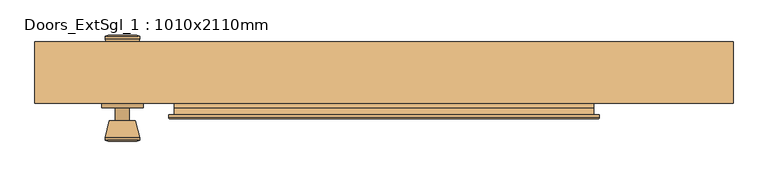
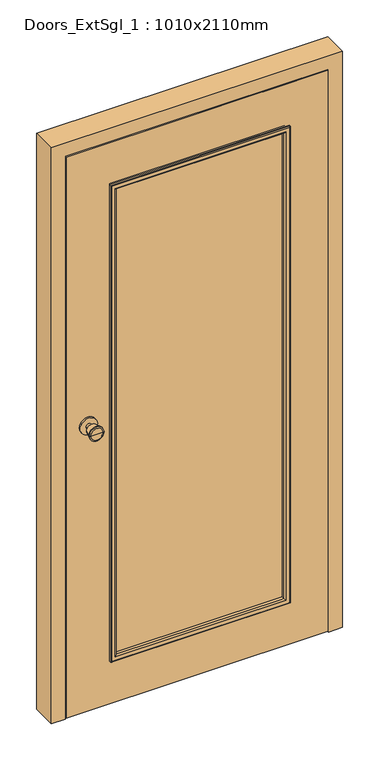
"""IFC4 building model written with IfcOpenShell, lengths in millimetres: door geometry, Doors_ExtSgl_1 : 1010x2110mm."""

from ifc_helpers import new_model, si_unit, point, frame, frame_2d, origin, place, context, project, spatial, polyline, circle_curve, ellipse_curve, trimmed, segment, composite_curve, outline, extrude, faceted_brep, source, transform, mapped, element, save
from ifc_brep_helpers import plane_surface, cylinder_surface, revolved_surface, advanced_brep


def doors_extsgl_1_1010x2110mm_099c12f8(model_context):
    return source(origin(), model_context, "Body", "SolidModel", [
        advanced_brep(
        [(-378.5, 46.25, 1050.0), (-368.5, 46.25, 1050.0), (-388.5, 46.25, 1050.0), (-358.0241324, -2.75, 1050.0), (-378.5, -2.75, 1050.0), (-398.9758676, -2.75, 1050.0), (-353.5, -0.9221319, 1050.0), (-403.5, -0.9221319, 1050.0), (-353.5, 2.5415463, 1050.0), (-403.5, 2.5415463, 1050.0), (-359.863764, 27.25, 1050.0), (-397.136236, 27.25, 1050.0), (-368.5, 27.25, 1050.0), (-388.5, 27.25, 1050.0)],
        [
            (0, 1),
            (1, 2, circle_curve(frame((-378.5, 46.25, 1050.0), z_axis=(0.0, 1.0, 0.0), x_axis=(-1.0, 0.0, 0.0)), 10.0)),
            (2, 0),
            (2, 1, circle_curve(frame((-378.5, 46.25, 1050.0), z_axis=(0.0, 1.0, 0.0), x_axis=(-1.0, 0.0, 0.0)), 10.0)),
            (3, 4),
            (4, 5),
            (5, 3, circle_curve(frame((-378.5, -2.75, 1050.0), z_axis=(0.0, -1.0, 0.0), x_axis=(-1.0, 0.0, 0.0)), 20.4758676)),
            (3, 5, circle_curve(frame((-378.5, -2.75, 1050.0), z_axis=(0.0, -1.0, 0.0), x_axis=(-1.0, 0.0, 0.0)), 20.4758676)),
            (6, 3),
            (5, 7),
            (7, 6, circle_curve(frame((-378.5, -0.9221319, 1050.0), z_axis=(0.0, -1.0, 0.0), x_axis=(-1.0, 0.0, 0.0)), 25.0)),
            (6, 7, circle_curve(frame((-378.5, -0.9221319, 1050.0), z_axis=(0.0, -1.0, 0.0), x_axis=(-1.0, 0.0, 0.0)), 25.0)),
            (8, 6),
            (7, 9),
            (9, 8, circle_curve(frame((-378.5, 2.5415463, 1050.0), z_axis=(0.0, -1.0, 0.0), x_axis=(-1.0, 0.0, 0.0)), 25.0)),
            (8, 9, circle_curve(frame((-378.5, 2.5415463, 1050.0), z_axis=(0.0, -1.0, 0.0), x_axis=(-1.0, 0.0, 0.0)), 25.0)),
            (10, 8),
            (9, 11),
            (11, 10, circle_curve(frame((-378.5, 27.25, 1050.0), z_axis=(0.0, -1.0, 0.0), x_axis=(-1.0, 0.0, 0.0)), 18.636236)),
            (10, 11, circle_curve(frame((-378.5, 27.25, 1050.0), z_axis=(0.0, -1.0, 0.0), x_axis=(-1.0, 0.0, 0.0)), 18.636236)),
            (12, 10),
            (11, 13),
            (13, 12, circle_curve(frame((-378.5, 27.25, 1050.0), z_axis=(0.0, -1.0, 0.0), x_axis=(-1.0, 0.0, 0.0)), 10.0)),
            (12, 13, circle_curve(frame((-378.5, 27.25, 1050.0), z_axis=(0.0, -1.0, 0.0), x_axis=(-1.0, 0.0, 0.0)), 10.0)),
            (1, 12),
            (13, 2),
        ],
        [
            plane_surface(frame((-378.5, 46.25, 1050.0), z_axis=(0.0, 1.0, 0.0), x_axis=(-1.0, 0.0, 0.0))),
            plane_surface(frame((-378.5, -2.75, 1050.0), z_axis=(0.0, -1.0, 0.0), x_axis=(-1.0, 0.0, 0.0))),
            revolved_surface(polyline([(-398.9758676, -2.75, 1050.0), (-403.5, -0.9221319, 1050.0)]), (-378.5, 46.25, 1050.0), (0.0, 1.0, 0.0)),
            cylinder_surface(frame((-378.5, 46.25, 1050.0), z_axis=(0.0, 1.0, 0.0), x_axis=(-1.0, 0.0, 0.0)), 25.0),
            revolved_surface(polyline([(-403.5, 2.5415463, 1050.0), (-397.136236, 27.25, 1050.0)]), (-378.5, 46.25, 1050.0), (0.0, 1.0, 0.0)),
            plane_surface(frame((-378.5, 27.25, 1050.0), z_axis=(0.0, 1.0, 0.0), x_axis=(-1.0, 0.0, 0.0))),
            cylinder_surface(frame((-378.5, 46.25, 1050.0), z_axis=(0.0, 1.0, 0.0), x_axis=(-1.0, 0.0, 0.0)), 10.0),
        ],
        [
            (0, [[1, 2, 3]]),
            (0, [[-3, 4, -1]]),
            (1, [[5, 6, 7]]),
            (1, [[-6, -5, 8]]),
            (2, [[9, -7, 10, 11]]),
            (2, [[-10, -8, -9, 12]]),
            (3, [[13, -11, 14, 15]]),
            (3, [[-14, -12, -13, 16]]),
            (4, [[17, -15, 18, 19]]),
            (4, [[-18, -16, -17, 20]]),
            (5, [[21, -19, 22, 23]]),
            (5, [[-22, -20, -21, 24]]),
            (6, [[25, -23, 26, -2]]),
            (6, [[-26, -24, -25, -4]]),
        ],
    ),
        extrude(outline(composite_curve([segment(trimmed(circle_curve(frame_2d((1050.0, -378.5)), 30.0), [point((1050.0, -408.5))], [point((1050.0, -348.5))], False, "CARTESIAN"), True, "CONTINUOUS"), segment(trimmed(circle_curve(frame_2d((1050.0, -378.5)), 30.0), [point((1050.0, -348.5))], [point((1050.0, -408.5))], False, "CARTESIAN"), True, "CONTINUOUS")], self_intersect=False)), frame((0.0, 46.25, 0.0), z_axis=(0.0, 1.0, 0.0), x_axis=(0.0, 0.0, 1.0)), (0.0, 0.0, 1.0), 6.0),
        advanced_brep(
        [(-378.5, 102.25, 1050.0), (-388.5, 102.25, 1050.0), (-368.5, 102.25, 1050.0), (-358.0241324, 151.25, 1050.0), (-398.9758676, 151.25, 1050.0), (-378.5, 151.25, 1050.0), (-353.5, 149.4221319, 1050.0), (-403.5, 149.4221319, 1050.0), (-353.5, 145.9584537, 1050.0), (-403.5, 145.9584537, 1050.0), (-359.863764, 121.25, 1050.0), (-397.136236, 121.25, 1050.0), (-368.5, 121.25, 1050.0), (-388.5, 121.25, 1050.0)],
        [
            (0, 1),
            (1, 2, circle_curve(frame((-378.5, 102.25, 1050.0), z_axis=(0.0, -1.0, 0.0), x_axis=(-1.0, 0.0, 0.0)), 10.0)),
            (2, 0),
            (2, 1, circle_curve(frame((-378.5, 102.25, 1050.0), z_axis=(0.0, -1.0, 0.0), x_axis=(-1.0, 0.0, 0.0)), 10.0)),
            (3, 4, circle_curve(frame((-378.5, 151.25, 1050.0), z_axis=(0.0, 1.0, 0.0), x_axis=(-1.0, 0.0, 0.0)), 20.4758676)),
            (4, 5),
            (5, 3),
            (4, 3, circle_curve(frame((-378.5, 151.25, 1050.0), z_axis=(0.0, 1.0, 0.0), x_axis=(-1.0, 0.0, 0.0)), 20.4758676)),
            (6, 7, circle_curve(frame((-378.5, 149.4221319, 1050.0), z_axis=(0.0, 1.0, 0.0), x_axis=(-1.0, 0.0, 0.0)), 25.0)),
            (7, 4),
            (3, 6),
            (7, 6, circle_curve(frame((-378.5, 149.4221319, 1050.0), z_axis=(0.0, 1.0, 0.0), x_axis=(-1.0, 0.0, 0.0)), 25.0)),
            (8, 9, circle_curve(frame((-378.5, 145.9584537, 1050.0), z_axis=(0.0, 1.0, 0.0), x_axis=(-1.0, 0.0, 0.0)), 25.0)),
            (9, 7),
            (6, 8),
            (9, 8, circle_curve(frame((-378.5, 145.9584537, 1050.0), z_axis=(0.0, 1.0, 0.0), x_axis=(-1.0, 0.0, 0.0)), 25.0)),
            (10, 11, circle_curve(frame((-378.5, 121.25, 1050.0), z_axis=(0.0, 1.0, 0.0), x_axis=(-1.0, 0.0, 0.0)), 18.636236)),
            (11, 9),
            (8, 10),
            (11, 10, circle_curve(frame((-378.5, 121.25, 1050.0), z_axis=(0.0, 1.0, 0.0), x_axis=(-1.0, 0.0, 0.0)), 18.636236)),
            (12, 13, circle_curve(frame((-378.5, 121.25, 1050.0), z_axis=(0.0, 1.0, 0.0), x_axis=(-1.0, 0.0, 0.0)), 10.0)),
            (13, 11),
            (10, 12),
            (13, 12, circle_curve(frame((-378.5, 121.25, 1050.0), z_axis=(0.0, 1.0, 0.0), x_axis=(-1.0, 0.0, 0.0)), 10.0)),
            (1, 13),
            (12, 2),
        ],
        [
            plane_surface(frame((-378.5, 102.25, 1050.0), z_axis=(0.0, -1.0, 0.0), x_axis=(-1.0, 0.0, 0.0))),
            plane_surface(frame((-378.5, 151.25, 1050.0), z_axis=(0.0, 1.0, 0.0), x_axis=(-1.0, 0.0, 0.0))),
            revolved_surface(polyline([(-398.9758676, 151.25, 1050.0), (-403.5, 149.4221319, 1050.0)]), (-378.5, 102.25, 1050.0), (0.0, -1.0, 0.0)),
            cylinder_surface(frame((-378.5, 102.25, 1050.0), z_axis=(0.0, -1.0, 0.0), x_axis=(-1.0, 0.0, 0.0)), 25.0),
            revolved_surface(polyline([(-403.5, 145.9584537, 1050.0), (-397.136236, 121.25, 1050.0)]), (-378.5, 102.25, 1050.0), (0.0, -1.0, 0.0)),
            plane_surface(frame((-378.5, 121.25, 1050.0), z_axis=(0.0, -1.0, 0.0), x_axis=(-1.0, 0.0, 0.0))),
            cylinder_surface(frame((-378.5, 102.25, 1050.0), z_axis=(0.0, -1.0, 0.0), x_axis=(-1.0, 0.0, 0.0)), 10.0),
        ],
        [
            (0, [[1, 2, 3]]),
            (0, [[-3, 4, -1]]),
            (1, [[5, 6, 7]]),
            (1, [[8, -7, -6]]),
            (2, [[9, 10, -5, 11]]),
            (2, [[12, -11, -8, -10]]),
            (3, [[13, 14, -9, 15]]),
            (3, [[16, -15, -12, -14]]),
            (4, [[17, 18, -13, 19]]),
            (4, [[20, -19, -16, -18]]),
            (5, [[21, 22, -17, 23]]),
            (5, [[24, -23, -20, -22]]),
            (6, [[-2, 25, -21, 26]]),
            (6, [[-4, -26, -24, -25]]),
        ],
    ),
        extrude(outline(composite_curve([segment(trimmed(circle_curve(frame_2d((1050.0, -378.5)), 30.0), [point((1050.0, -408.5))], [point((1050.0, -348.5))], False, "CARTESIAN"), True, "CONTINUOUS"), segment(trimmed(circle_curve(frame_2d((1050.0, -378.5)), 30.0), [point((1050.0, -348.5))], [point((1050.0, -408.5))], False, "CARTESIAN"), True, "CONTINUOUS")], self_intersect=False)), frame((0.0, 96.25, 0.0), z_axis=(0.0, 1.0, 0.0), x_axis=(0.0, 0.0, 1.0)), (0.0, 0.0, 1.0), 6.0),
        faceted_brep([(434.5, 141.25, 0.0), (505.0, 141.25, 0.0), (505.0, 52.25, 0.0), (456.5, 52.25, 0.0), (456.5, 99.25, 0.0), (434.5, 99.25, 0.0), (434.5, 141.25, 2039.5), (-434.5, 141.25, 2039.5), (-434.5, 141.25, 0.0), (-505.0, 141.25, 0.0), (-505.0, 141.25, 2110.0), (505.0, 141.25, 2110.0), (505.0, 52.25, 2110.0), (-505.0, 52.25, 2110.0), (-505.0, 52.25, 0.0), (-456.5, 52.25, 0.0), (-456.5, 52.25, 2061.5), (456.5, 52.25, 2061.5), (456.5, 99.25, 2061.5), (-456.5, 99.25, 2061.5), (-456.5, 99.25, 0.0), (-434.5, 99.25, 0.0), (-434.5, 99.25, 2039.5), (434.5, 99.25, 2039.5)], [[[0, 1, 2, 3, 4, 5]], [[1, 0, 6, 7, 8, 9, 10, 11]], [[2, 1, 11, 12]], [[3, 2, 12, 13, 14, 15, 16, 17]], [[4, 3, 17, 18]], [[5, 4, 18, 19, 20, 21, 22, 23]], [[0, 5, 23, 6]], [[7, 22, 21, 8]], [[8, 21, 20, 15, 14, 9]], [[13, 10, 9, 14]], [[19, 16, 15, 20]], [[12, 11, 10, 13]], [[18, 17, 16, 19]], [[6, 23, 22, 7]]]),
        extrude(outline(polyline([(-303.5, 70.0), (303.5, 70.0), (303.5, 46.0), (-303.5, 46.0), (-303.5, 70.0)])), frame((0.0, 0.0, 179.0), z_axis=(0.0, 0.0, 1.0), x_axis=(1.0, 0.0, 0.0)), (0.0, 0.0, 1.0), 1729.5),
        extrude(outline(polyline([(4.0, 453.5), (2058.5, 453.5), (2058.5, -454.4250294), (4.0, -454.4250294), (4.0, 453.5)]), holes=[polyline([(179.0, -303.5), (1908.5, -303.5), (1908.5, 303.5), (179.0, 303.5), (179.0, -303.5)])]), frame((0.0, 52.25, 0.0), z_axis=(0.0, 1.0, 0.0), x_axis=(0.0, 0.0, 1.0)), (0.0, 0.0, 1.0), 44.0),
        advanced_brep(
        [(311.5, 32.0, 171.0), (311.5, 36.0, 171.0), (311.5, 36.0, 1916.5), (311.5, 32.0, 1916.5), (309.5, 30.0, 173.0), (309.5, 30.0, 1914.5), (291.5, 35.0, 191.0), (296.5, 30.0, 186.0), (296.5, 30.0, 1901.5), (291.5, 35.0, 1896.5), (291.5, 46.0, 191.0), (291.5, 46.0, 1896.5), (303.5, 36.0, 179.0), (303.5, 46.0, 179.0), (303.5, 46.0, 1908.5), (303.5, 36.0, 1908.5), (-311.5, 36.0, 1916.5), (-311.5, 32.0, 1916.5), (-309.5, 30.0, 1914.5), (-296.5, 30.0, 1901.5), (-291.5, 35.0, 1896.5), (-291.5, 46.0, 1896.5), (-303.5, 46.0, 1908.5), (-303.5, 36.0, 1908.5), (-311.5, 36.0, 171.0), (-311.5, 32.0, 171.0), (-309.5, 30.0, 173.0), (-296.5, 30.0, 186.0), (-291.5, 35.0, 191.0), (-291.5, 46.0, 191.0), (-303.5, 46.0, 179.0), (-303.5, 36.0, 179.0)],
        [
            (0, 1),
            (1, 2),
            (2, 3),
            (3, 0),
            (4, 0, ellipse_curve(frame((309.5, 32.0, 173.0), z_axis=(0.7071067811865475, 0.0, 0.7071067811865476), x_axis=(0.7071067811865476, 0.0, -0.7071067811865475)), 2.8284271, 2.0)),
            (3, 5, ellipse_curve(frame((309.5, 32.0, 1914.5), z_axis=(0.7071067811865475, 0.0, -0.7071067811865475), x_axis=(-0.7071067811865474, 0.0, -0.7071067811865476)), 2.8284271, 2.0)),
            (5, 4),
            (6, 7, ellipse_curve(frame((296.5, 35.0, 186.0), z_axis=(0.7071067811865475, 0.0, 0.7071067811865476), x_axis=(0.7071067811865476, 0.0, -0.7071067811865475)), 7.0710678, 5.0)),
            (7, 8),
            (8, 9, ellipse_curve(frame((296.5, 35.0, 1901.5), z_axis=(0.7071067811865475, 0.0, -0.7071067811865475), x_axis=(-0.7071067811865474, 0.0, -0.7071067811865476)), 7.0710678, 5.0)),
            (9, 6),
            (10, 6),
            (9, 11),
            (11, 10),
            (12, 13),
            (13, 14),
            (14, 15),
            (15, 12),
            (2, 16),
            (16, 17),
            (17, 3),
            (17, 18, ellipse_curve(frame((-309.5, 32.0, 1914.5), z_axis=(0.7071067811865476, 0.0, 0.7071067811865475), x_axis=(0.7071067811865474, 0.0, -0.7071067811865476)), 2.8284271, 2.0)),
            (18, 5),
            (8, 19),
            (19, 20, ellipse_curve(frame((-296.5, 35.0, 1901.5), z_axis=(0.7071067811865476, 0.0, 0.7071067811865475), x_axis=(0.7071067811865474, 0.0, -0.7071067811865476)), 7.0710678, 5.0)),
            (20, 9),
            (20, 21),
            (21, 11),
            (14, 22),
            (22, 23),
            (23, 15),
            (16, 24),
            (24, 25),
            (25, 17),
            (25, 26, ellipse_curve(frame((-309.5, 32.0, 173.0), z_axis=(-0.7071067811865475, 0.0, 0.7071067811865475), x_axis=(0.7071067811865474, 0.0, 0.7071067811865476)), 2.8284271, 2.0)),
            (26, 18),
            (19, 27),
            (27, 28, ellipse_curve(frame((-296.5, 35.0, 186.0), z_axis=(-0.7071067811865475, 0.0, 0.7071067811865475), x_axis=(0.7071067811865474, 0.0, 0.7071067811865476)), 7.0710678, 5.0)),
            (28, 20),
            (28, 29),
            (29, 21),
            (22, 30),
            (30, 31),
            (31, 23),
            (24, 1),
            (0, 25),
            (4, 26),
            (7, 27),
            (6, 28),
            (10, 29),
            (13, 30),
            (12, 31),
        ],
        [
            plane_surface(frame((311.5, 36.0, 171.0), z_axis=(1.0, 0.0, 0.0), x_axis=(0.0, 0.0, 1.0))),
            cylinder_surface(frame((309.5, 32.0, 179.0), z_axis=(0.0, 0.0, -1.0), x_axis=(1.0, 0.0, 0.0)), 2.0),
            cylinder_surface(frame((296.5, 35.0, 179.0), z_axis=(0.0, 0.0, -1.0), x_axis=(1.0, 0.0, 0.0)), 5.0),
            plane_surface(frame((291.5, 35.0, 191.0), z_axis=(-1.0, 0.0, 0.0), x_axis=(0.0, 0.0, 1.0))),
            plane_surface(frame((303.5, 46.0, 179.0), z_axis=(1.0, 0.0, 0.0), x_axis=(0.0, 0.0, 1.0))),
            plane_surface(frame((311.5, 36.0, 1916.5), z_axis=(0.0, 0.0, 1.0), x_axis=(-1.0, 0.0, 0.0))),
            cylinder_surface(frame((303.5, 32.0, 1914.5), z_axis=(1.0, 0.0, 0.0), x_axis=(0.0, 0.0, 1.0)), 2.0),
            cylinder_surface(frame((303.5, 35.0, 1901.5), z_axis=(1.0, 0.0, 0.0), x_axis=(0.0, 0.0, 1.0)), 5.0),
            plane_surface(frame((291.5, 35.0, 1896.5), z_axis=(0.0, 0.0, -1.0), x_axis=(-1.0, 0.0, 0.0))),
            plane_surface(frame((303.5, 46.0, 1908.5), z_axis=(0.0, 0.0, 1.0), x_axis=(-1.0, 0.0, 0.0))),
            plane_surface(frame((-311.5, 36.0, 1916.5), z_axis=(-1.0, 0.0, 0.0), x_axis=(0.0, 0.0, -1.0))),
            cylinder_surface(frame((-309.5, 32.0, 1908.5), z_axis=(0.0, 0.0, 1.0), x_axis=(-1.0, 0.0, 0.0)), 2.0),
            cylinder_surface(frame((-296.5, 35.0, 1908.5), z_axis=(0.0, 0.0, 1.0), x_axis=(-1.0, 0.0, 0.0)), 5.0),
            plane_surface(frame((-291.5, 35.0, 1896.5), z_axis=(1.0, 0.0, 0.0), x_axis=(0.0, 0.0, -1.0))),
            plane_surface(frame((-303.5, 46.0, 1908.5), z_axis=(-1.0, 0.0, 0.0), x_axis=(0.0, 0.0, -1.0))),
            plane_surface(frame((-311.5, 36.0, 171.0), z_axis=(0.0, 0.0, -1.0), x_axis=(1.0, 0.0, 0.0))),
            cylinder_surface(frame((-303.5, 32.0, 173.0), z_axis=(-1.0, 0.0, 0.0), x_axis=(0.0, 0.0, -1.0)), 2.0),
            plane_surface(frame((-309.5, 30.0, 173.0), z_axis=(0.0, -1.0, 0.0), x_axis=(1.0, 0.0, 0.0))),
            cylinder_surface(frame((-303.5, 35.0, 186.0), z_axis=(-1.0, 0.0, 0.0), x_axis=(0.0, 0.0, -1.0)), 5.0),
            plane_surface(frame((-291.5, 35.0, 191.0), z_axis=(0.0, 0.0, 1.0), x_axis=(1.0, 0.0, 0.0))),
            plane_surface(frame((-291.5, 46.0, 191.0), z_axis=(0.0, 1.0, 0.0), x_axis=(1.0, 0.0, 0.0))),
            plane_surface(frame((-303.5, 46.0, 179.0), z_axis=(0.0, 0.0, -1.0), x_axis=(1.0, 0.0, 0.0))),
            plane_surface(frame((-303.5, 36.0, 179.0), z_axis=(0.0, 1.0, 0.0), x_axis=(1.0, 0.0, 0.0))),
        ],
        [
            (0, [[1, 2, 3, 4]]),
            (1, [[5, -4, 6, 7]]),
            (2, [[8, 9, 10, 11]]),
            (3, [[12, -11, 13, 14]]),
            (4, [[15, 16, 17, 18]]),
            (5, [[-3, 19, 20, 21]]),
            (6, [[-6, -21, 22, 23]]),
            (7, [[-10, 24, 25, 26]]),
            (8, [[-13, -26, 27, 28]]),
            (9, [[-17, 29, 30, 31]]),
            (10, [[-20, 32, 33, 34]]),
            (11, [[-22, -34, 35, 36]]),
            (12, [[-25, 37, 38, 39]]),
            (13, [[-27, -39, 40, 41]]),
            (14, [[-30, 42, 43, 44]]),
            (15, [[-33, 45, -1, 46]]),
            (16, [[-35, -46, -5, 47]]),
            (17, [[-23, -36, -47, -7], [48, -37, -24, -9]]),
            (18, [[-38, -48, -8, 49]]),
            (19, [[-40, -49, -12, 50]]),
            (20, [[51, -42, -29, -16], [-28, -41, -50, -14]]),
            (21, [[-43, -51, -15, 52]]),
            (22, [[-45, -32, -19, -2], [-31, -44, -52, -18]]),
        ],
    ),
        advanced_brep(
        [(-311.5, 84.0, 171.0), (-311.5, 80.0, 171.0), (-311.5, 80.0, 1916.5), (-311.5, 84.0, 1916.5), (-309.5, 86.0, 173.0), (-309.5, 86.0, 1914.5), (-291.5, 81.0, 191.0), (-296.5, 86.0, 186.0), (-296.5, 86.0, 1901.5), (-291.5, 81.0, 1896.5), (-291.5, 70.0, 191.0), (-291.5, 70.0, 1896.5), (-303.5, 80.0, 179.0), (-303.5, 70.0, 179.0), (-303.5, 70.0, 1908.5), (-303.5, 80.0, 1908.5), (311.5, 80.0, 1916.5), (311.5, 84.0, 1916.5), (309.5, 86.0, 1914.5), (296.5, 86.0, 1901.5), (291.5, 81.0, 1896.5), (291.5, 70.0, 1896.5), (303.5, 70.0, 1908.5), (303.5, 80.0, 1908.5), (311.5, 80.0, 171.0), (311.5, 84.0, 171.0), (309.5, 86.0, 173.0), (296.5, 86.0, 186.0), (291.5, 81.0, 191.0), (291.5, 70.0, 191.0), (303.5, 70.0, 179.0), (303.5, 80.0, 179.0)],
        [
            (0, 1),
            (1, 2),
            (2, 3),
            (3, 0),
            (4, 0, ellipse_curve(frame((-309.5, 84.0, 173.0), z_axis=(-0.7071067811865475, 0.0, 0.7071067811865475), x_axis=(-0.7071067811865474, 0.0, -0.7071067811865476)), 2.8284271, 2.0)),
            (3, 5, ellipse_curve(frame((-309.5, 84.0, 1914.5), z_axis=(-0.7071067811865475, 0.0, -0.7071067811865475), x_axis=(0.7071067811865474, 0.0, -0.7071067811865476)), 2.8284271, 2.0)),
            (5, 4),
            (6, 7, ellipse_curve(frame((-296.5, 81.0, 186.0), z_axis=(-0.7071067811865475, 0.0, 0.7071067811865475), x_axis=(-0.7071067811865474, 0.0, -0.7071067811865476)), 7.0710678, 5.0)),
            (7, 8),
            (8, 9, ellipse_curve(frame((-296.5, 81.0, 1901.5), z_axis=(-0.7071067811865475, 0.0, -0.7071067811865475), x_axis=(0.7071067811865474, 0.0, -0.7071067811865476)), 7.0710678, 5.0)),
            (9, 6),
            (10, 6),
            (9, 11),
            (11, 10),
            (12, 13),
            (13, 14),
            (14, 15),
            (15, 12),
            (2, 16),
            (16, 17),
            (17, 3),
            (17, 18, ellipse_curve(frame((309.5, 84.0, 1914.5), z_axis=(-0.7071067811865475, 0.0, 0.7071067811865475), x_axis=(-0.7071067811865476, 0.0, -0.7071067811865474)), 2.8284271, 2.0)),
            (18, 5),
            (8, 19),
            (19, 20, ellipse_curve(frame((296.5, 81.0, 1901.5), z_axis=(-0.7071067811865475, 0.0, 0.7071067811865475), x_axis=(-0.7071067811865476, 0.0, -0.7071067811865474)), 7.0710678, 5.0)),
            (20, 9),
            (20, 21),
            (21, 11),
            (14, 22),
            (22, 23),
            (23, 15),
            (16, 24),
            (24, 25),
            (25, 17),
            (25, 26, ellipse_curve(frame((309.5, 84.0, 173.0), z_axis=(0.7071067811865476, 0.0, 0.7071067811865475), x_axis=(-0.7071067811865475, 0.0, 0.7071067811865476)), 2.8284271, 2.0)),
            (26, 18),
            (19, 27),
            (27, 28, ellipse_curve(frame((296.5, 81.0, 186.0), z_axis=(0.7071067811865476, 0.0, 0.7071067811865475), x_axis=(-0.7071067811865475, 0.0, 0.7071067811865476)), 7.0710678, 5.0)),
            (28, 20),
            (28, 29),
            (29, 21),
            (22, 30),
            (30, 31),
            (31, 23),
            (24, 1),
            (0, 25),
            (4, 26),
            (7, 27),
            (6, 28),
            (10, 29),
            (13, 30),
            (12, 31),
        ],
        [
            plane_surface(frame((-311.5, 80.0, 171.0), z_axis=(-1.0, 0.0, 0.0), x_axis=(0.0, 0.0, 1.0))),
            cylinder_surface(frame((-309.5, 84.0, 179.0), z_axis=(0.0, 0.0, -1.0), x_axis=(-1.0, 0.0, 0.0)), 2.0),
            cylinder_surface(frame((-296.5, 81.0, 179.0), z_axis=(0.0, 0.0, -1.0), x_axis=(-1.0, 0.0, 0.0)), 5.0),
            plane_surface(frame((-291.5, 81.0, 191.0), z_axis=(1.0, 0.0, 0.0), x_axis=(0.0, 0.0, 1.0))),
            plane_surface(frame((-303.5, 70.0, 179.0), z_axis=(-1.0, 0.0, 0.0), x_axis=(0.0, 0.0, 1.0))),
            plane_surface(frame((-311.5, 80.0, 1916.5), z_axis=(0.0, 0.0, 1.0), x_axis=(1.0, 0.0, 0.0))),
            cylinder_surface(frame((-303.5, 84.0, 1914.5), z_axis=(-1.0, 0.0, 0.0), x_axis=(0.0, 0.0, 1.0)), 2.0),
            cylinder_surface(frame((-303.5, 81.0, 1901.5), z_axis=(-1.0, 0.0, 0.0), x_axis=(0.0, 0.0, 1.0)), 5.0),
            plane_surface(frame((-291.5, 81.0, 1896.5), z_axis=(0.0, 0.0, -1.0), x_axis=(1.0, 0.0, 0.0))),
            plane_surface(frame((-303.5, 70.0, 1908.5), z_axis=(0.0, 0.0, 1.0), x_axis=(1.0, 0.0, 0.0))),
            plane_surface(frame((311.5, 80.0, 1916.5), z_axis=(1.0, 0.0, 0.0), x_axis=(0.0, 0.0, -1.0))),
            cylinder_surface(frame((309.5, 84.0, 1908.5), z_axis=(0.0, 0.0, 1.0), x_axis=(1.0, 0.0, 0.0)), 2.0),
            cylinder_surface(frame((296.5, 81.0, 1908.5), z_axis=(0.0, 0.0, 1.0), x_axis=(1.0, 0.0, 0.0)), 5.0),
            plane_surface(frame((291.5, 81.0, 1896.5), z_axis=(-1.0, 0.0, 0.0), x_axis=(0.0, 0.0, -1.0))),
            plane_surface(frame((303.5, 70.0, 1908.5), z_axis=(1.0, 0.0, 0.0), x_axis=(0.0, 0.0, -1.0))),
            plane_surface(frame((311.5, 80.0, 171.0), z_axis=(0.0, 0.0, -1.0), x_axis=(-1.0, 0.0, 0.0))),
            cylinder_surface(frame((303.5, 84.0, 173.0), z_axis=(1.0, 0.0, 0.0), x_axis=(0.0, 0.0, -1.0)), 2.0),
            plane_surface(frame((309.5, 86.0, 173.0), z_axis=(0.0, 1.0, 0.0), x_axis=(-1.0, 0.0, 0.0))),
            cylinder_surface(frame((303.5, 81.0, 186.0), z_axis=(1.0, 0.0, 0.0), x_axis=(0.0, 0.0, -1.0)), 5.0),
            plane_surface(frame((291.5, 81.0, 191.0), z_axis=(0.0, 0.0, 1.0), x_axis=(-1.0, 0.0, 0.0))),
            plane_surface(frame((291.5, 70.0, 191.0), z_axis=(0.0, -1.0, 0.0), x_axis=(-1.0, 0.0, 0.0))),
            plane_surface(frame((303.5, 70.0, 179.0), z_axis=(0.0, 0.0, -1.0), x_axis=(-1.0, 0.0, 0.0))),
            plane_surface(frame((303.5, 80.0, 179.0), z_axis=(0.0, -1.0, 0.0), x_axis=(-1.0, 0.0, 0.0))),
        ],
        [
            (0, [[1, 2, 3, 4]]),
            (1, [[5, -4, 6, 7]]),
            (2, [[8, 9, 10, 11]]),
            (3, [[12, -11, 13, 14]]),
            (4, [[15, 16, 17, 18]]),
            (5, [[-3, 19, 20, 21]]),
            (6, [[-6, -21, 22, 23]]),
            (7, [[-10, 24, 25, 26]]),
            (8, [[-13, -26, 27, 28]]),
            (9, [[-17, 29, 30, 31]]),
            (10, [[-20, 32, 33, 34]]),
            (11, [[-22, -34, 35, 36]]),
            (12, [[-25, 37, 38, 39]]),
            (13, [[-27, -39, 40, 41]]),
            (14, [[-30, 42, 43, 44]]),
            (15, [[-33, 45, -1, 46]]),
            (16, [[-35, -46, -5, 47]]),
            (17, [[-23, -36, -47, -7], [48, -37, -24, -9]]),
            (18, [[-38, -48, -8, 49]]),
            (19, [[-40, -49, -12, 50]]),
            (20, [[51, -42, -29, -16], [-28, -41, -50, -14]]),
            (21, [[-43, -51, -15, 52]]),
            (22, [[-45, -32, -19, -2], [-31, -44, -52, -18]]),
        ],
    ),
    ])


if __name__ == "__main__":
    model = new_model("IFC4")
    model_context = context("Model", 3, world=origin())
    ifc_project = project(units=[si_unit("LENGTHUNIT", "METRE", prefix="MILLI")], contexts=[model_context])
    site = spatial("IfcSite", under=ifc_project)
    building = spatial("IfcBuilding", under=site)
    placement = place(None, origin())
    doors_extsgl_1_1010x2110mm_shape = doors_extsgl_1_1010x2110mm_099c12f8(model_context)
    element("IfcDoor", 1, ObjectType="Doors_ExtSgl_1 : 1010x2110mm", at=placement, inside=building, context=model_context, shape_type="MappedRepresentation", body=[
        mapped(doors_extsgl_1_1010x2110mm_shape, transform((0.0, 0.0, 0.0), x_axis=(1.0, 0.0, 0.0), y_axis=(0.0, 1.0, 0.0), z_axis=(0.0, 0.0, 1.0))),
    ])
    save(model, "model.ifc")

# Revit data of these elements
# Type "Doors_ExtSgl_1 : 1010x2110mm"
#   Type Mark = "72"
#   Type Comments = "External Single"
#   Operation = "SingleSwingRight"
#   Construction Type Id = "SGL"
#   Keynote = "L20"
#   Analytic Construction = "Large single-glazed windows"
#   Wrap Layers (Int) from Ext = 177.5 mm
#   Wrap Layers (Ext) from Ext = 102.5 mm
#   Visual Light Transmittance = 0.9
#   Thickness = 44 mm
#   Stile Shutting = 150 mm
#   Stile - Top Rail = 150 mm
#   Stile - Hanging = 150 mm
#   Stile - Bottom Rail = 175 mm
#   Solar Heat Gain Coefficient = 0.86
#   Rough Width = 1010 mm
#   Rough Height = 2110 mm
#   O/A Frame Width = 64 mm
#   Heat Transfer Coefficient (U) = 5.5617 W/(m²·K)
#   Handle Z Distance = 1050 mm
#   Glazing Thickness = 24 mm
#   Glazing Bar Thickness = 20 mm
#   FrameWidth = 42 mm
#   FrameOffset - External = 25 mm
#   FrameDepth = 89 mm
#   Door Panel Width = 907 mm
#   Handle X Distance = 75 mm
#   Height = 2110 mm
#   Structural Tolerance = 6.5 mm
#   Tolerance = 3 mm
#   Undercut = 4 mm
#   Width = 1010 mm
#   Door Panel Thickness = 44 mm
#   Door Panel Height = 2054.5 mm
#   Cavity Closer Width = 50 mm
#   Cavity Closer Offset from Ext = 102.5 mm
#   Cavity Closer Depth = 85 mm
#   Vis - Ironmongery = yes
#   Vis - Cavity Closers = yes
#   Define Thermal Properties by = 1
#   Function = 1
#   Material Glass = Door - Glazing
#   Handle Style = element 939899
#   Material Door = Door - Panel
#   Material Frame = Door - Frame/Mullion
#   Material Ironmongery = Door - Handle
#   Wall Closure = (empty or 0)
# Element 1 (IfcDoor, "Doors_ExtSgl_1 : 1010x2110mm")
#   Materials on its faces: "Door - Panel", "Door - Handle", "Door - Frame/Mullion", "Door - Glazing"
# Materials
#   "Door - Glazing": class "Miscellaneous", colour RGB 0 0 255, transparency 0.75
#   "Door - Panel": class "Wood", colour RGB 210 159 95, transparency 0, Keynote = "L20"
#   "Door - Frame/Mullion": class "Wood", colour RGB 212 179 113, transparency 0, Keynote = "L20"
#   "Door - Handle": class "Miscellaneous", colour RGB 0 0 0, transparency 0, Keynote = "P21"
